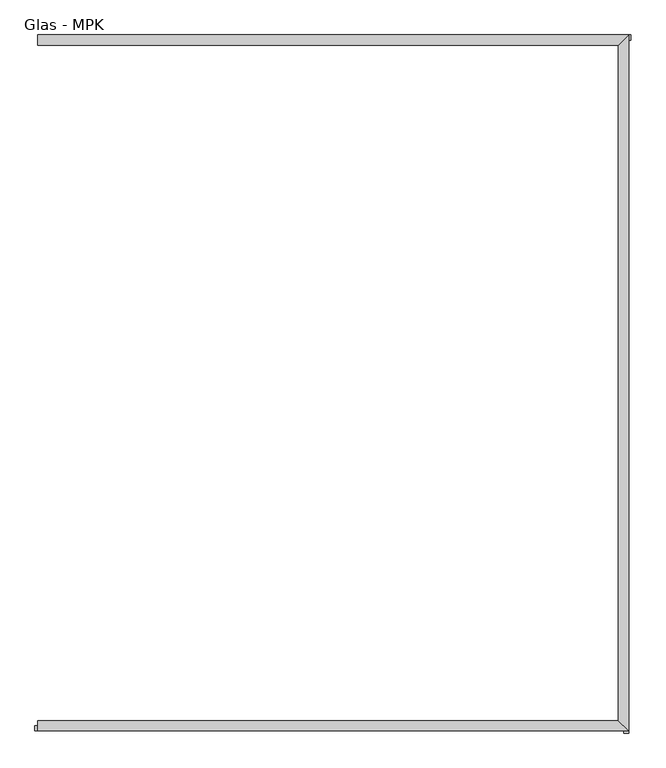
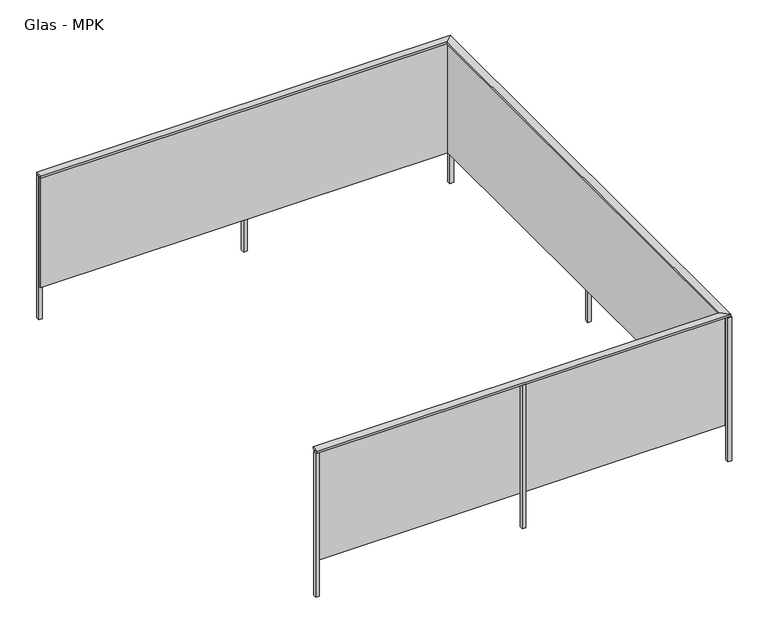
"""IFC4 building model written with IfcOpenShell, lengths in millimetres: railing geometry, Glas - MPK."""

from ifc_helpers import new_model, si_unit, frame, origin, place, context, project, spatial, polyline, outline, extrude, faceted_brep, source, transform, mapped, element, save


def glas_mpk_39525c5c(model_context):
    return source(origin(), model_context, "Body", "SolidModel", [
        faceted_brep([(28810.8437289, 1285.374085, 9843.2628643), (28810.8437289, 1235.374085, 9843.2628643), (28810.8437289, 1235.374085, 9856.7371357), (28810.8437289, 1285.374085, 9856.7371357), (31650.8437289, 1285.374085, 9843.2628643), (31600.8437289, 1235.374085, 9843.2628643), (31600.8437289, 1235.374085, 9856.7371357), (31650.8437289, 1285.374085, 9856.7371357), (31650.8437289, -2055.3552612, 9843.2628643), (31600.8437289, -2005.3552612, 9843.2628643), (31600.8437289, -2005.3552612, 9856.7371357), (31650.8437289, -2055.3552612, 9856.7371357), (28810.8437289, -2055.3552612, 9843.2628643), (28810.8437289, -2055.3552612, 9856.7371357), (28810.8437289, -2005.3552612, 9856.7371357), (28810.8437289, -2005.3552612, 9843.2628643)], [[[0, 1, 2, 3]], [[1, 0, 4, 5]], [[2, 1, 5, 6]], [[3, 2, 6, 7]], [[0, 3, 7, 4]], [[5, 4, 8, 9]], [[6, 5, 9, 10]], [[7, 6, 10, 11]], [[4, 7, 11, 8]], [[12, 13, 14, 15]], [[9, 8, 12, 15]], [[10, 9, 15, 14]], [[11, 10, 14, 13]], [[8, 11, 13, 12]]]),
        faceted_brep([(28810.8437289, 1245.374085, 9842.8769824), (28810.8437289, 1259.566209, 9842.8769824), (28810.8437289, 1259.566209, 9042.8769824), (28810.8437289, 1245.374085, 9042.8769824), (31610.8437289, 1245.374085, 9842.8769824), (31625.0358529, 1259.566209, 9842.8769824), (31625.0358529, 1259.566209, 9042.8769824), (31610.8437289, 1245.374085, 9042.8769824), (31610.8437289, -2015.3552612, 9842.8769824), (31625.0358529, -2029.5473852, 9842.8769824), (31625.0358529, -2029.5473852, 9042.8769824), (31610.8437289, -2015.3552612, 9042.8769824), (28810.8437289, -2015.3552612, 9842.8769824), (28810.8437289, -2015.3552612, 9042.8769824), (28810.8437289, -2029.5473852, 9042.8769824), (28810.8437289, -2029.5473852, 9842.8769824)], [[[0, 1, 2, 3]], [[1, 0, 4, 5]], [[2, 1, 5, 6]], [[3, 2, 6, 7]], [[0, 3, 7, 4]], [[5, 4, 8, 9]], [[6, 5, 9, 10]], [[7, 6, 10, 11]], [[4, 7, 11, 8]], [[12, 13, 14, 15]], [[9, 8, 12, 15]], [[10, 9, 15, 14]], [[11, 10, 14, 13]], [[8, 11, 13, 12]]]),
        extrude(outline(polyline([(30242.0937289, -2030.3552612), (30242.0937289, -2055.3552612), (30217.0937289, -2055.3552612), (30217.0937289, -2030.3552612), (30242.0937289, -2030.3552612)])), frame((0.0, 0.0, 8800.0), z_axis=(0.0, 0.0, 1.0), x_axis=(1.0, 0.0, 0.0)), (0.0, 0.0, 1.0), 1043.2628643),
        extrude(outline(polyline([(31625.8437289, -372.4905881), (31650.8437289, -372.4905881), (31650.8437289, -397.4905881), (31625.8437289, -397.4905881), (31625.8437289, -372.4905881)])), frame((0.0, 0.0, 8800.0), z_axis=(0.0, 0.0, 1.0), x_axis=(1.0, 0.0, 0.0)), (0.0, 0.0, 1.0), 1043.2628643),
        extrude(outline(polyline([(30217.0937289, 1260.374085), (30217.0937289, 1285.374085), (30242.0937289, 1285.374085), (30242.0937289, 1260.374085), (30217.0937289, 1260.374085)])), frame((0.0, 0.0, 8800.0), z_axis=(0.0, 0.0, 1.0), x_axis=(1.0, 0.0, 0.0)), (0.0, 0.0, 1.0), 1043.2628643),
        extrude(outline(polyline([(31625.8437289, -2040.3552612), (31650.8437289, -2040.3552612), (31650.8437289, -2065.3552612), (31625.8437289, -2065.3552612), (31625.8437289, -2040.3552612)])), frame((0.0, 0.0, 8800.0), z_axis=(0.0, 0.0, 1.0), x_axis=(1.0, 0.0, 0.0)), (0.0, 0.0, 1.0), 1043.2628643),
        extrude(outline(polyline([(31635.8437289, 1260.374085), (31635.8437289, 1285.374085), (31660.8437289, 1285.374085), (31660.8437289, 1260.374085), (31635.8437289, 1260.374085)])), frame((0.0, 0.0, 8800.0), z_axis=(0.0, 0.0, 1.0), x_axis=(1.0, 0.0, 0.0)), (0.0, 0.0, 1.0), 1043.2628643),
        extrude(outline(polyline([(28823.3437289, -2030.3552612), (28823.3437289, -2055.3552612), (28798.3437289, -2055.3552612), (28798.3437289, -2030.3552612), (28823.3437289, -2030.3552612)])), frame((0.0, 0.0, 8800.0), z_axis=(0.0, 0.0, 1.0), x_axis=(1.0, 0.0, 0.0)), (0.0, 0.0, 1.0), 1043.2628643),
        extrude(outline(polyline([(28810.8437289, 1260.374085), (28810.8437289, 1285.374085), (28835.8437289, 1285.374085), (28835.8437289, 1260.374085), (28810.8437289, 1260.374085)])), frame((0.0, 0.0, 8800.0), z_axis=(0.0, 0.0, 1.0), x_axis=(1.0, 0.0, 0.0)), (0.0, 0.0, 1.0), 1043.2628643),
    ])


if __name__ == "__main__":
    model = new_model("IFC4")
    model_context = context("Model", 3, world=origin())
    ifc_project = project(units=[si_unit("LENGTHUNIT", "METRE", prefix="MILLI")], contexts=[model_context])
    site = spatial("IfcSite", under=ifc_project)
    building = spatial("IfcBuilding", under=site)
    placement = place(None, origin())
    glas_mpk_shape = glas_mpk_39525c5c(model_context)
    element("IfcRailing", 1, ObjectType="Glas - MPK", at=placement, inside=building, context=model_context, shape_type="MappedRepresentation", body=[
        mapped(glas_mpk_shape, transform((0.0, 0.0, 0.0), x_axis=(1.0, 0.0, 0.0), y_axis=(0.0, 1.0, 0.0), z_axis=(0.0, 0.0, 1.0))),
    ])
    save(model, "model.ifc")

# Revit data of these elements
# Element 1 (IfcRailing, "Glas - MPK")
#   Materials on its faces: "Metal - Aluminum", "Window - Glass"
# Materials
#   "Metal - Aluminum": class "Unassigned", colour RGB 247 247 247, transparency 0, Comments = "Rendering appearance not upgraded "
#   "Window - Glass": class "Glas", colour RGB 128 128 255, transparency 0.75
